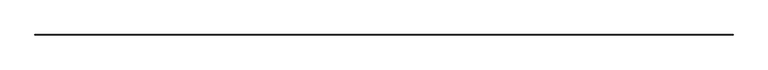
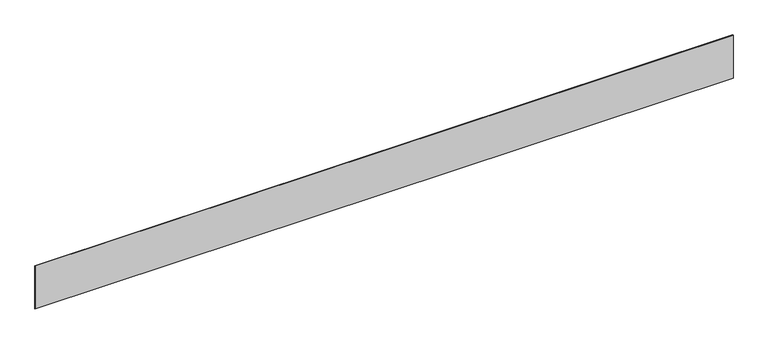
"""IFC4 building model written with IfcOpenShell, lengths in millimetres: proxy geometry, Inner panel:Inner panel:1:Inner panel:1 : Inner panel:Inner panel:300324:300043:Inner panel:1:Inner panel:1 : Inner panel:Inner panel:300324:300043 : Inner panel:Inner panel:1:Inner panel:1 : Inner panel:Inner panel:300324:300043:34 : Inner panel:Inner panel:1:Inner panel:1 : Inner panel:Inner panel:300324:300043:Inner panel:1:Inner panel:1 : Inner panel:Inner panel:300324:300043 : Inner panel:Inner panel:1:Inner panel:1 : Inner panel:Inner panel:300324:300043:300031."""

import ifcopenshell
import ifcopenshell.guid

model = None  # the IFC model being written
_history = None  # IfcOwnerHistory: only IFC2X3 demands one
_inside = {}  # id of a spatial element -> (the spatial element, [elements in it])
_under = {}  # id of a project, library or spatial element -> (it, [spatial elements below it])
_declared = {}  # id of a project -> (the project, [libraries it declares])
_typed = {}  # id of a type object -> (the type object, [elements of that type])
_made_of = {}  # id of a material, layer set ... -> (it, [elements and type objects made of it])


def new_model(schema):
    """Start an empty IFC model of exactly this schema.

    Asked for "IFC4X3", IfcOpenShell would pick the latest addendum, in which some entities
    have other attributes; the version numbers below select the first issue.
    IFC2X3 requires an IfcOwnerHistory on every rooted entity: one is made here for all.
    """
    global model, _history
    if schema == "IFC4X3":
        model = ifcopenshell.file(schema_version=(4, 3, 0, 0))
    else:
        model = ifcopenshell.file(schema=schema)
    _inside.clear()
    _under.clear()
    _declared.clear()
    _typed.clear()
    _made_of.clear()
    _history = None
    if model.schema == "IFC2X3":
        org = make("IfcOrganization", Name="unknown")
        user = make(
            "IfcPersonAndOrganization",
            ThePerson=make("IfcPerson", FamilyName="unknown"),
            TheOrganization=org,
        )
        app = make(
            "IfcApplication",
            ApplicationDeveloper=org,
            Version="unknown",
            ApplicationFullName="unknown",
            ApplicationIdentifier="unknown",
        )
        _history = make(
            "IfcOwnerHistory",
            OwningUser=user,
            OwningApplication=app,
            ChangeAction="ADDED",
            CreationDate=0,
        )
    return model


def make(cls, **values):
    """One entity of the class cls with the attributes given. An attribute that is None is left unset."""
    return model.create_entity(
        cls, **{name: value for name, value in values.items() if value is not None}
    )


def rooted(cls, **values):
    """An entity with a GlobalId (a new one), such as an element, a storey or a relation."""
    return make(cls, GlobalId=ifcopenshell.guid.new(), OwnerHistory=_history, **values)


def si_unit(unit_type, name, prefix=None):
    """IfcSIUnit, for example si_unit("LENGTHUNIT", "METRE", prefix="MILLI")."""
    return make("IfcSIUnit", UnitType=unit_type, Prefix=prefix, Name=name)


def assignment(units):
    """IfcUnitAssignment: the units of a project."""
    return None if units is None else make("IfcUnitAssignment", Units=units)


def point(xyz):
    """IfcCartesianPoint."""
    return None if xyz is None else make("IfcCartesianPoint", Coordinates=xyz)


def direction(xyz):
    """IfcDirection."""
    return None if xyz is None else make("IfcDirection", DirectionRatios=xyz)


def frame(location, z_axis=None, x_axis=None):
    """IfcAxis2Placement3D, a coordinate frame: its origin and axes. An axis left out is left unset."""
    return make(
        "IfcAxis2Placement3D",
        Location=point(location),
        Axis=direction(z_axis),
        RefDirection=direction(x_axis),
    )


def origin():
    """The frame at (0, 0, 0) with its axes left unset."""
    return frame((0.0, 0.0, 0.0))


def place(relative_to, where):
    """IfcLocalPlacement: puts the frame where relative to a parent placement (None: the world)."""
    return make(
        "IfcLocalPlacement", PlacementRelTo=relative_to, RelativePlacement=where
    )


def context(
    kind, dimensions, precision=None, world=None, true_north=None, identifier=None
):
    """IfcGeometricRepresentationContext, for example the 3D "Model" context."""
    return make(
        "IfcGeometricRepresentationContext",
        ContextIdentifier=identifier,
        ContextType=kind,
        CoordinateSpaceDimension=dimensions,
        Precision=precision,
        WorldCoordinateSystem=world,
        TrueNorth=true_north,
    )


def project(units=None, contexts=None):
    """IfcProject with its units and contexts."""
    return rooted(
        "IfcProject",
        Name="project",
        RepresentationContexts=contexts,
        UnitsInContext=assignment(units),
    )


def spatial(cls, under=None, at=None, **own):
    """A site, building, storey or space (cls), placed at a placement, below another one or the project."""
    s = rooted(cls, ObjectPlacement=at, **own)
    if under is not None:
        _under.setdefault(under.id(), (under, []))[1].append(s)
    return s


def polyline(points):
    """IfcPolyline through the points."""
    return make("IfcPolyline", Points=[point(p) for p in points])


def outline(outer, holes=None, kind="AREA"):
    """IfcArbitraryClosedProfileDef: a profile drawn as a closed curve; with holes, ...WithVoids."""
    if holes is None:
        return make("IfcArbitraryClosedProfileDef", ProfileType=kind, OuterCurve=outer)
    return make(
        "IfcArbitraryProfileDefWithVoids",
        ProfileType=kind,
        OuterCurve=outer,
        InnerCurves=holes,
    )


def extrude(swept, where, along, depth):
    """IfcExtrudedAreaSolid: the profile swept, set in the frame where, extruded along a direction by depth."""
    return make(
        "IfcExtrudedAreaSolid",
        SweptArea=swept,
        Position=where,
        ExtrudedDirection=direction(along),
        Depth=depth,
    )


def shape(context_of_items, identifier, shape_type, items):
    """IfcShapeRepresentation: the items that make up one representation, for example the "Body"."""
    return make(
        "IfcShapeRepresentation",
        ContextOfItems=context_of_items,
        RepresentationIdentifier=identifier,
        RepresentationType=shape_type,
        Items=items,
    )


def source(mapping_origin, context_of_items, identifier, shape_type, items):
    """IfcRepresentationMap: a shape defined once, which mapped items show again and again."""
    return make(
        "IfcRepresentationMap",
        MappingOrigin=mapping_origin,
        MappedRepresentation=shape(context_of_items, identifier, shape_type, items),
    )


def transform(
    local_origin,
    x_axis=None,
    y_axis=None,
    z_axis=None,
    scale=None,
    scale2=None,
    scale3=None,
    uniform=True,
):
    """IfcCartesianTransformationOperator3D, or its non-uniform kind. x_axis, y_axis, z_axis: its Axis1, 2, 3."""
    if uniform:
        return make(
            "IfcCartesianTransformationOperator3D",
            Axis1=direction(x_axis),
            Axis2=direction(y_axis),
            LocalOrigin=point(local_origin),
            Scale=scale,
            Axis3=direction(z_axis),
        )
    return make(
        "IfcCartesianTransformationOperator3DnonUniform",
        Axis1=direction(x_axis),
        Axis2=direction(y_axis),
        LocalOrigin=point(local_origin),
        Scale=scale,
        Axis3=direction(z_axis),
        Scale2=scale2,
        Scale3=scale3,
    )


def mapped(mapping_source, mapping_target):
    """IfcMappedItem: shows the shape of a source again, moved by a transform."""
    return make(
        "IfcMappedItem", MappingSource=mapping_source, MappingTarget=mapping_target
    )


def made_of(thing, what):
    """Note that an element or type object is made of a material, layer set ...; save() writes the relation."""
    if what is not None:
        _made_of.setdefault(what.id(), (what, []))[1].append(thing)
    return thing


def element(
    cls,
    number,
    at=None,
    inside=None,
    cuts=None,
    type_object=None,
    material=None,
    context=None,
    identifier="Body",
    shape_type=None,
    held_by="IfcProductDefinitionShape",
    body=None,
    shapes=None,
    **own,
):
    """One element of the class cls, such as IfcWall. Its Tag is "e" and its number.

    at: its placement. inside: the storey or other place that contains it. cuts: it is an
    opening in that element (IfcRelVoidsElement). A single representation is given by context,
    identifier, shape_type and body (its items); several are given by shapes. held_by: the class
    of the entity that holds the representations. save() writes the other relations.
    """
    e = rooted(cls, Tag="e%d" % number, ObjectPlacement=at, **own)
    if body is not None:
        shapes = [shape(context, identifier, shape_type, body)]
    if shapes is not None:
        e.Representation = make(held_by, Representations=shapes)
    if inside is not None:
        _inside.setdefault(inside.id(), (inside, []))[1].append(e)
    if cuts is not None:
        rooted(
            "IfcRelVoidsElement", RelatingBuildingElement=cuts, RelatedOpeningElement=e
        )
    if type_object is not None:
        _typed.setdefault(type_object.id(), (type_object, []))[1].append(e)
    return made_of(e, material)


def aggregate(whole, parts):
    """IfcRelAggregates: a whole, such as a stair, and the parts it consists of."""
    return rooted("IfcRelAggregates", RelatingObject=whole, RelatedObjects=parts)


def save(model, path):
    """Write the relations noted so far, then the file.

    IfcRelAggregates (storeys below a building ...), IfcRelContainedInSpatialStructure (elements
    in a storey), IfcRelDefinesByType, IfcRelAssociatesMaterial and IfcRelDeclares: one each for
    every whole, place, type object, material and project.
    """
    for whole, parts in _under.values():
        aggregate(whole, parts)
    for where, things in _inside.values():
        rooted(
            "IfcRelContainedInSpatialStructure",
            RelatedElements=things,
            RelatingStructure=where,
        )
    for kind, things in _typed.values():
        rooted("IfcRelDefinesByType", RelatedObjects=things, RelatingType=kind)
    for what, things in _made_of.values():
        rooted("IfcRelAssociatesMaterial", RelatedObjects=things, RelatingMaterial=what)
    for by, libraries in _declared.values():
        rooted("IfcRelDeclares", RelatingContext=by, RelatedDefinitions=libraries)
    model.write(path)


def generic_models_4dca0cbf(model_context):
    return source(origin(), model_context, "Body", "SweptSolid", [
        extrude(outline(polyline([(560648.236724, -579000.6913841), (579307.7117239, -579000.6913841), (579307.7117239, -579013.3913841), (560648.236724, -579013.3913841), (560648.236724, -579000.6913841)])), frame((0.0, 0.0, 4946.65), z_axis=(0.0, 0.0, 1.0), x_axis=(1.0, 0.0, 0.0)), (0.0, 0.0, 1.0), 1219.2),
    ])


if __name__ == "__main__":
    model = new_model("IFC4")
    model_context = context("Model", 3, world=origin())
    ifc_project = project(units=[si_unit("LENGTHUNIT", "METRE", prefix="MILLI")], contexts=[model_context])
    site = spatial("IfcSite", under=ifc_project)
    building = spatial("IfcBuilding", under=site)
    placement = place(None, origin())
    generic_models_shape = generic_models_4dca0cbf(model_context)
    element("IfcBuildingElementProxy", 1, Name="Inner panel:Inner panel:1:Inner panel:1 : Inner panel:Inner panel:300324:300043:Inner panel:1:Inner panel:1 : Inner panel:Inner panel:300324:300043 : Inner panel:Inner panel:1:Inner panel:1 : Inner panel:Inner panel:300324:300043:34 : Inner panel:Inner panel:1:Inner panel:1 : Inner panel:Inner panel:300324:300043:Inner panel:1:Inner panel:1 : Inner panel:Inner panel:300324:300043 : Inner panel:Inner panel:1:Inner panel:1 : Inner panel:Inner panel:300324:300043:300031", ObjectType="Inner panel:Inner panel:1:Inner panel:1 : Inner panel:Inner panel:300324:300043:Inner panel:1:Inner panel:1 : Inner panel:Inner panel:300324:300043 : Inner panel:Inner panel:1:Inner panel:1 : Inner panel:Inner panel:300324:300043:34 : Inner panel:Inner panel:1:Inner panel:1 : Inner panel:Inner panel:300324:300043:Inner panel:1:Inner panel:1 : Inner panel:Inner panel:300324:300043 : Inner panel:Inner panel:1:Inner panel:1 : Inner panel:Inner panel:300324:300043:300031", at=placement, inside=building, context=model_context, shape_type="MappedRepresentation", body=[
        mapped(generic_models_shape, transform((0.0, 0.0, 0.0), x_axis=(1.0, 0.0, 0.0), y_axis=(0.0, 1.0, 0.0), z_axis=(0.0, 0.0, 1.0))),
    ])
    save(model, "model.ifc")

# Revit data of these elements
# Type "Inner panel:Inner panel:1:Inner panel:1 : Inner panel:Inner panel:300324:300043:Inner panel:1:Inner panel:1 : Inner panel:Inner panel:300324:300043 : Inner panel:Inner panel:1:Inner panel:1 : Inner panel:Inner panel:300324:300043:34 : Inner panel:Inner panel:1:Inner panel:1 : Inner panel:Inner panel:300324:300043:Inner panel:1:Inner panel:1 : Inner panel:Inner panel:300324:300043 : Inner panel:Inner panel:1:Inner panel:1 : Inner panel:Inner panel:300324:300043:300031"
#   NameOverride = "Inner panel:Inner panel:1:Inner panel:1 : Inner panel:Inner panel:300324:300043:Inner panel:1:Inner panel:1 : Inner panel:Inner panel:300324:300043 : Inner panel:Inner panel:1:Inner panel:1 : Inner panel:Inner panel:300324:300043:300031"
#   ObjectTypeOverride = "Inner panel:1:Inner panel:1 : Inner panel:Inner panel:300324:300043 : Inner panel:Inner panel:1:Inner panel:1 : Inner panel:Inner panel:300324:300043"
#   Reference = "Inner panel"
#   Tag = "300031"
# Element 1 (IfcBuildingElementProxy, "Inner panel:Inner panel:1:Inner panel:1 : Inner panel:Inner panel:300324:300043:Inner panel:1:Inner panel:1 : Inner panel:Inner panel:300324:300043 : Inner panel:Inner panel:1:Inner panel:1 : Inner panel:Inner panel:300324:300043:34 : Inner panel:Inner panel:1:Inner panel:1 : Inner panel:Inner panel:300324:300043:Inner panel:1:Inner panel:1 : Inner panel:Inner panel:300324:300043 : Inner panel:Inner panel:1:Inner panel:1 : Inner panel:Inner panel:300324:300043:300031")
#   Materials on its faces: "1/2\" FIBERGLASS MAT GYPSUM PANELS"
# Materials
#   "1/2\" FIBERGLASS MAT GYPSUM PANELS": class "Generic", colour RGB 171 170 168, transparency 0, Description = "Gypsum Wall Board", Cost = 0
